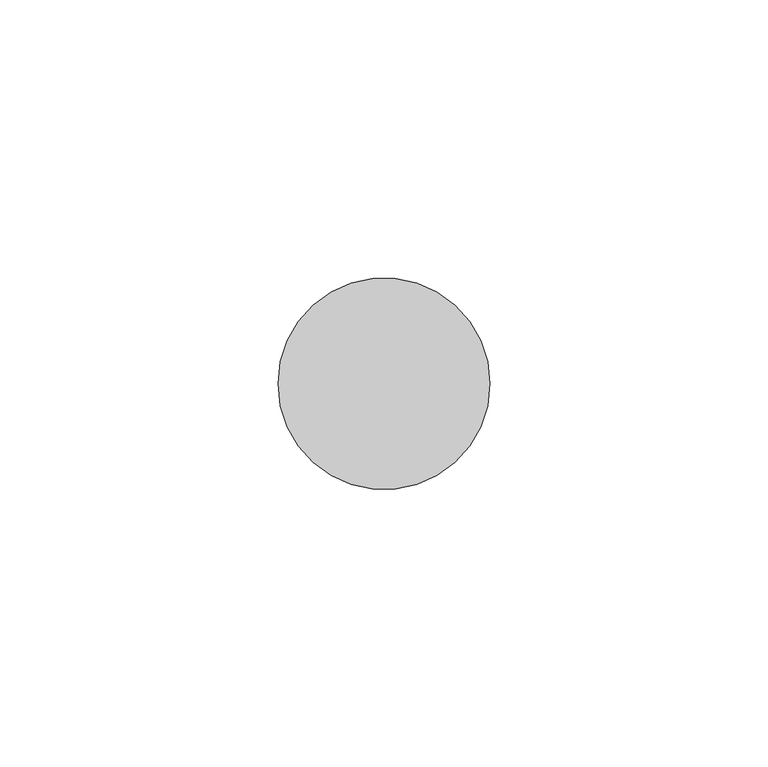
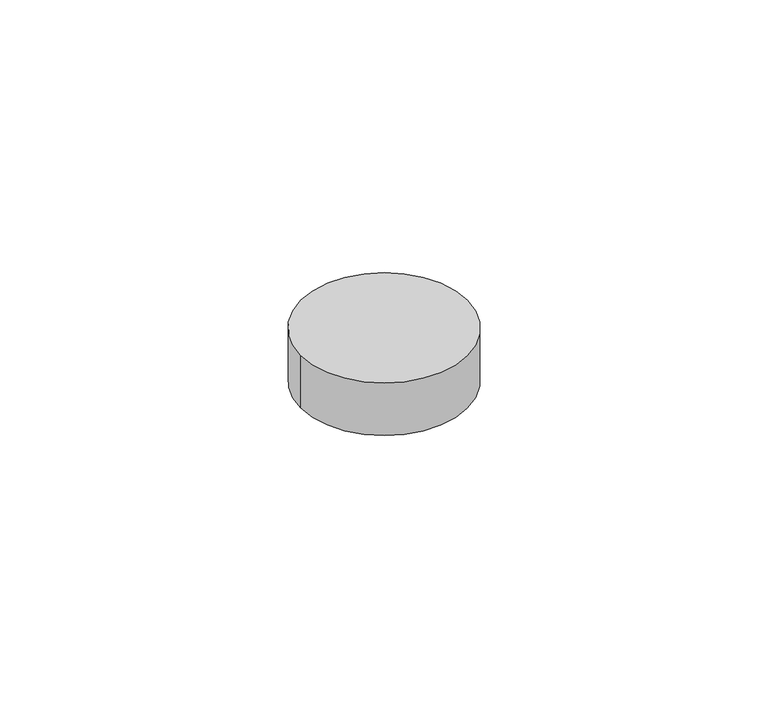
"""IFC4 building model written with IfcOpenShell, lengths in millimetres: proxy geometry, Bolt002 8688 : Bolt002 8688."""

from ifc_helpers import new_model, si_unit, point, frame, frame_2d, origin, place, context, project, spatial, circle_curve, trimmed, segment, composite_curve, outline, extrude, source, transform, mapped, element, save


def generic_models_b789c14b(model_context):
    return source(origin(), model_context, "Body", "SweptSolid", [
        extrude(outline(composite_curve([segment(trimmed(circle_curve(frame_2d((7415.2612305, -1781.8449707)), 19.05), [point((7396.2112305, -1781.8449707))], [point((7434.3112305, -1781.8449707))], False, "CARTESIAN"), True, "CONTINUOUS"), segment(trimmed(circle_curve(frame_2d((7415.2612305, -1781.8449707)), 19.05), [point((7434.3112305, -1781.8449707))], [point((7396.2112305, -1781.8449707))], False, "CARTESIAN"), True, "CONTINUOUS")], self_intersect=False)), frame((0.0, 0.0, 40112.696), z_axis=(0.0, 0.0, 1.0), x_axis=(1.0, 0.0, 0.0)), (0.0, 0.0, 1.0), 12.7),
    ])


if __name__ == "__main__":
    model = new_model("IFC4")
    model_context = context("Model", 3, world=origin())
    ifc_project = project(units=[si_unit("LENGTHUNIT", "METRE", prefix="MILLI")], contexts=[model_context])
    site = spatial("IfcSite", under=ifc_project)
    building = spatial("IfcBuilding", under=site)
    placement = place(None, origin())
    generic_models_shape = generic_models_b789c14b(model_context)
    element("IfcBuildingElementProxy", 1, Name="Bolt002 8688 : Bolt002 8688", ObjectType="Bolt002 8688 : Bolt002 8688", at=placement, inside=building, context=model_context, shape_type="MappedRepresentation", body=[
        mapped(generic_models_shape, transform((0.0, 0.0, 0.0), x_axis=(1.0, 0.0, 0.0), y_axis=(0.0, 1.0, 0.0), z_axis=(0.0, 0.0, 1.0))),
    ])
    save(model, "model.ifc")

# Revit data of these elements
# Type "Bolt002 8688 : Bolt002 8688"
#   NameOverride = "Bolt002"
# Element 1 (IfcBuildingElementProxy, "Bolt002 8688 : Bolt002 8688")
#   Materials on its faces: "BOLTS CONCEALED BY FLOOR FINISH"
# Materials
#   "BOLTS CONCEALED BY FLOOR FINISH": class "Unassigned", colour RGB 128 128 128, transparency 0
